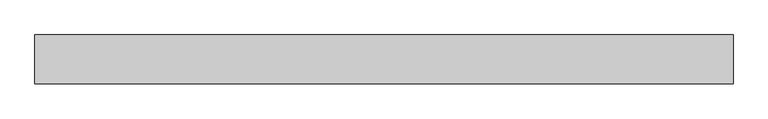
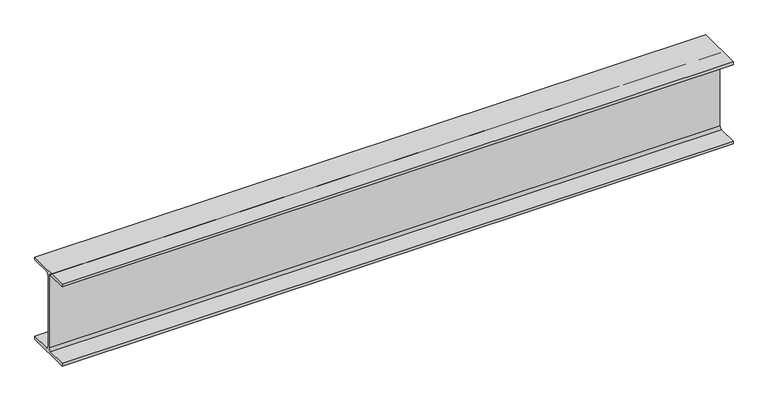
"""IFC4 building model written with IfcOpenShell, lengths in millimetres: beam geometry, Steel Beam_H-KSD3502 : H_SB_ASB_H-200x200x8x12."""

from ifc_helpers import new_model, si_unit, point, frame, frame_2d, origin, place, context, project, spatial, polyline, circle_curve, trimmed, segment, composite_curve, outline, extrude, source, transform, mapped, element, save


def beam_bc7b9760(model_context):
    return source(origin(), model_context, "Body", "SweptSolid", [
        extrude(outline(composite_curve([segment(polyline([(82.5, -141.5), (82.5, -151.7), (-82.5, -151.7), (-82.5, -141.5), (-11.9, -141.5)]), True, "CONTINUOUS"), segment(trimmed(circle_curve(frame_2d((-11.9, -132.6)), 8.9), [point((-11.9, -141.5))], [point((-3.0, -132.6))], True, "CARTESIAN"), True, "CONTINUOUS"), segment(polyline([(-3.0, -132.6), (-3.0, 132.6)]), True, "CONTINUOUS"), segment(trimmed(circle_curve(frame_2d((-11.9, 132.6)), 8.9), [point((-3.0, 132.6))], [point((-11.9, 141.5))], True, "CARTESIAN"), True, "CONTINUOUS"), segment(polyline([(-11.9, 141.5), (-82.5, 141.5), (-82.5, 151.7), (82.5, 151.7), (82.5, 141.5), (11.9, 141.5)]), True, "CONTINUOUS"), segment(trimmed(circle_curve(frame_2d((11.9, 132.6)), 8.9), [point((11.9, 141.5))], [point((3.0, 132.6))], True, "CARTESIAN"), True, "CONTINUOUS"), segment(polyline([(3.0, 132.6), (3.0, -132.6)]), True, "CONTINUOUS"), segment(trimmed(circle_curve(frame_2d((11.9, -132.6)), 8.9), [point((3.0, -132.6))], [point((11.9, -141.5))], True, "CARTESIAN"), True, "CONTINUOUS"), segment(polyline([(11.9, -141.5), (82.5, -141.5)]), True, "CONTINUOUS")], self_intersect=False)), frame((-1166.1355565, 0.0, 0.0), z_axis=(1.0, 0.0, 0.0), x_axis=(0.0, 1.0, 0.0)), (0.0, 0.0, 1.0), 2350.5623426),
    ])


if __name__ == "__main__":
    model = new_model("IFC4")
    model_context = context("Model", 3, world=origin())
    ifc_project = project(units=[si_unit("LENGTHUNIT", "METRE", prefix="MILLI")], contexts=[model_context])
    site = spatial("IfcSite", under=ifc_project)
    building = spatial("IfcBuilding", under=site)
    placement = place(None, origin())
    beam_shape = beam_bc7b9760(model_context)
    element("IfcBeam", 1, ObjectType="Steel Beam_H-KSD3502 : H_SB_ASB_H-200x200x8x12", at=placement, inside=building, context=model_context, shape_type="MappedRepresentation", body=[
        mapped(beam_shape, transform((0.0, 0.0, 0.0), x_axis=(1.0, 0.0, 0.0), y_axis=(0.0, 1.0, 0.0), z_axis=(0.0, 0.0, 1.0))),
    ])
    save(model, "model.ifc")

# Revit data of these elements
# Type "Steel Beam_H-KSD3502 : H_SB_ASB_H-200x200x8x12"
#   Width = 20.0 cm
#   Web Thickness = 0.8 cm
#   Web Fillet = 1.3 cm
#   Warping Constant = 141376.0 cm⁶
#   Torsional Moment of Inertia = 26.2485 cm⁴
#   Torsional Modulus = 1.0 cm³
#   Section Area = 63.53 cm²
#   Plastic Modulus weak axis = 244.0 cm³
#   Plastic Modulus strong axis = 525.0 cm³
#   Perimeter = 1.16 m²/m
#   Nominal Weight = 49.90 kgf/m
#   Moment of Inertia weak axis = 1600.00 cm⁴
#   Moment of Inertia strong axis = 4720.00 cm⁴
#   Height = 20.0 cm
#   Flange Thickness = 1.2 cm
#   Elastic Modulus weak axis = 160.0 cm³
#   Elastic Modulus strong axis = 472.0 cm³
#   Centroid Vertical = 10.0 cm
#   Centroid Horizontal = 10.0 cm
#   Length [instance default] = 1.5240 m
#   Structural Material [instance default] = Steel, 45-345
#   Assembly Code = ""
# Element 1 (IfcBeam, "Steel Beam_H-KSD3502 : H_SB_ASB_H-200x200x8x12")
#   Structural Material = none
# Materials
#   "Steel, 45-345": class "Metal", colour RGB 189 187 185, transparency 0, Description = "Steel 345 MPa", Cost = 0
